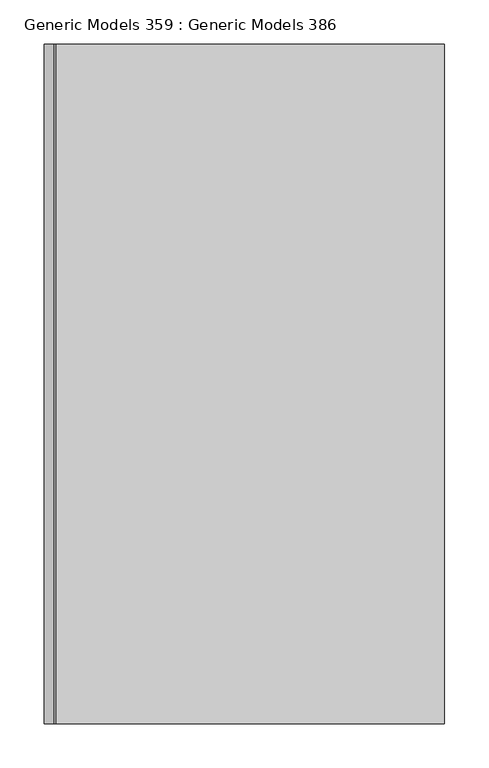
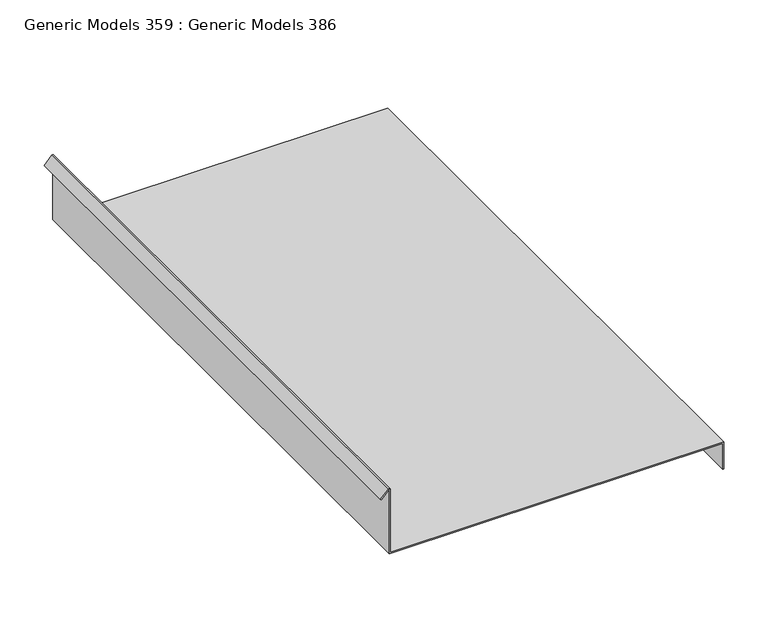
"""IFC4 building model written with IfcOpenShell, lengths in millimetres: proxy geometry, Generic Models 359 : Generic Models 386."""

from ifc_helpers import new_model, si_unit, point, frame, frame_2d, origin, place, context, project, spatial, polyline, circle_curve, trimmed, segment, composite_curve, outline, extrude, source, transform, mapped, element, save


def generic_models_359_generic_models_386_b65c5137(model_context):
    return source(origin(), model_context, "Body", "SweptSolid", [
        extrude(outline(composite_curve([segment(polyline([(127247.4498353, -6627.0096898), (127247.4498353, -7064.4438133), (127334.8936456, -7064.4438133)]), True, "CONTINUOUS"), segment(trimmed(circle_curve(frame_2d((127334.8936456, -7065.8485908)), 1.4047775), [point((127334.8936456, -7064.4438133))], [point((127335.8869733, -7066.8419185))], False, "CARTESIAN"), True, "CONTINUOUS"), segment(polyline([(127335.8869733, -7066.8419185), (127325.5400705, -7077.1888212), (127324.6280133, -7076.276764), (127335.1711201, -7065.7336571), (127246.1599915, -7065.7336571), (127246.1599915, -6628.2995335), (127210.1921566, -6628.2995335), (127210.1921566, -6627.0096898), (127247.4498353, -6627.0096898)]), True, "CONTINUOUS")], self_intersect=False)), frame((0.0, -4250.542257, 0.0), z_axis=(0.0, 1.0, 0.0), x_axis=(0.0, 0.0, 1.0)), (0.0, 0.0, 1.0), 763.8192232),
    ])


if __name__ == "__main__":
    model = new_model("IFC4")
    model_context = context("Model", 3, world=origin())
    ifc_project = project(units=[si_unit("LENGTHUNIT", "METRE", prefix="MILLI")], contexts=[model_context])
    site = spatial("IfcSite", under=ifc_project)
    building = spatial("IfcBuilding", under=site)
    placement = place(None, origin())
    generic_models_359_generic_models_386_shape = generic_models_359_generic_models_386_b65c5137(model_context)
    element("IfcBuildingElementProxy", 1, Name="Generic Models 359 : Generic Models 386", ObjectType="Generic Models 359 : Generic Models 386", at=placement, inside=building, context=model_context, shape_type="MappedRepresentation", body=[
        mapped(generic_models_359_generic_models_386_shape, transform((0.0, 0.0, 0.0), x_axis=(1.0, 0.0, 0.0), y_axis=(0.0, 1.0, 0.0), z_axis=(0.0, 0.0, 1.0))),
    ])
    save(model, "model.ifc")

# Revit data of these elements
# Element 1 (IfcBuildingElementProxy, "Generic Models 359 : Generic Models 386")
#   Materials on its faces: "_16 GA. COPPER BRAKE METAL FASCIA"
# Materials
#   "_16 GA. COPPER BRAKE METAL FASCIA": class "Generic", colour RGB 175 175 175, transparency 0, Cost = 0
